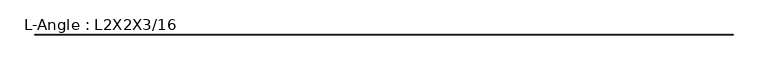
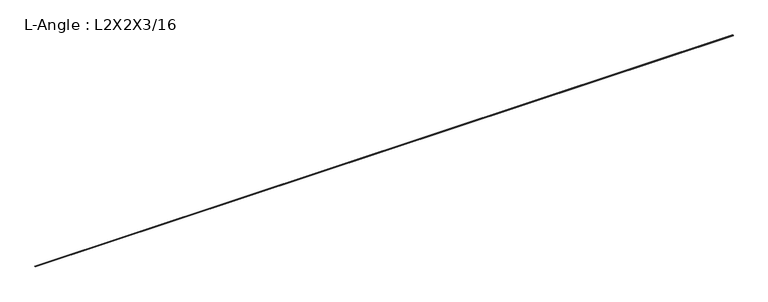
"""IFC4 building model written with IfcOpenShell, lengths in millimetres: beam geometry, L-Angle : L2X2X3/16."""

from ifc_helpers import new_model, si_unit, point, frame, frame_2d, origin, place, context, project, spatial, polyline, circle_curve, trimmed, segment, composite_curve, outline, extrude, source, transform, mapped, element, save


def l_angle_l2x2x3_16_9da130ac(model_context):
    return source(origin(), model_context, "Body", "SweptSolid", [
        extrude(outline(composite_curve([segment(polyline([(-14.2494, 14.2494), (36.5506, 14.2494)]), True, "CONTINUOUS"), segment(trimmed(circle_curve(frame_2d((31.7881, 14.2494)), 4.7625), [point((36.5506, 14.2494))], [point((31.7881, 9.4869))], False, "CARTESIAN"), True, "CONTINUOUS"), segment(polyline([(31.7881, 9.4869), (-4.7244, 9.4869)]), True, "CONTINUOUS"), segment(trimmed(circle_curve(frame_2d((-4.7244, 4.7244)), 4.7625), [point((-4.7244, 9.4869))], [point((-9.4869, 4.7244))], True, "CARTESIAN"), True, "CONTINUOUS"), segment(polyline([(-9.4869, 4.7244), (-9.4869, -31.7881)]), True, "CONTINUOUS"), segment(trimmed(circle_curve(frame_2d((-14.2494, -31.7881)), 4.7625), [point((-9.4869, -31.7881))], [point((-14.2494, -36.5506))], False, "CARTESIAN"), True, "CONTINUOUS"), segment(polyline([(-14.2494, -36.5506), (-14.2494, 14.2494)]), True, "CONTINUOUS")], self_intersect=False)), frame((-44322.7519531, 0.0, 0.0), z_axis=(1.0, 0.0, 0.0), x_axis=(0.0, 1.0, 0.0)), (0.0, 0.0, 1.0), 88645.5039063),
    ])


if __name__ == "__main__":
    model = new_model("IFC4")
    model_context = context("Model", 3, world=origin())
    ifc_project = project(units=[si_unit("LENGTHUNIT", "METRE", prefix="MILLI")], contexts=[model_context])
    site = spatial("IfcSite", under=ifc_project)
    building = spatial("IfcBuilding", under=site)
    placement = place(None, origin())
    l_angle_l2x2x3_16_shape = l_angle_l2x2x3_16_9da130ac(model_context)
    element("IfcBeam", 1, ObjectType="L-Angle : L2X2X3/16", at=placement, inside=building, context=model_context, shape_type="MappedRepresentation", body=[
        mapped(l_angle_l2x2x3_16_shape, transform((0.0, 0.0, 0.0), x_axis=(1.0, 0.0, 0.0), y_axis=(0.0, 1.0, 0.0), z_axis=(0.0, 0.0, 1.0))),
    ])
    save(model, "model.ifc")

# Revit data of these elements
# Type "L-Angle : L2X2X3/16"
#   Assembly Code = "B10"
#   k = 0' - 0 7/16"
#   W = 2.44
#   Start Extension Calculation [instance default] = 10' - 0"
#   Start Extension [instance default] = -0' - 0 1/2"
#   End Extension Calculation [instance default] = 10' - 0"
#   End Extension [instance default] = -0' - 0 1/2"
#   Length [instance default] = 5' - 0"
#   b = 0' - 2"
#   d = 0' - 2"
#   t = 0' - 0 3/16"
#   x = 0' - 0.561"
#   y = 0' - 0.561"
#   A = 0.00496528 SF
#   Structural Material [instance default] = Metal - Steel - ASTM A36
# Element 1 (IfcBeam, "L-Angle : L2X2X3/16")
#   Structural Material = STRUCTURAL STEEL - SEE STRUCT. DWGS
#   Materials on its faces: "STRUCTURAL STEEL - SEE STRUCT. DWGS"
# Materials
#   "Metal - Steel - ASTM A36": class "Metal", colour RGB 199 199 199, transparency 0
#   "STRUCTURAL STEEL - SEE STRUCT. DWGS": class "Metal", colour RGB 137 146 153, transparency 0, Description = "Steel, mill finish", Cost = 0
